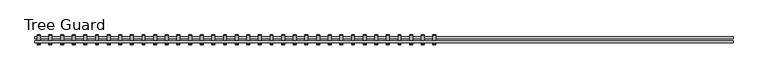
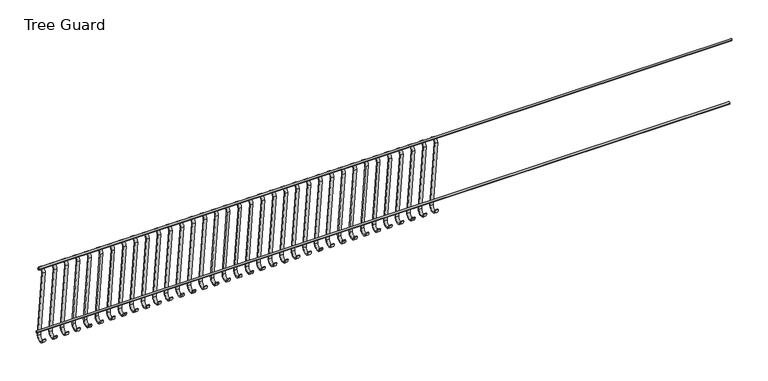
"""IFC4 building model written with IfcOpenShell, lengths in millimetres: railing geometry, Tree Guard."""

import ifcopenshell
import ifcopenshell.guid

model = None  # the IFC model being written
_history = None  # IfcOwnerHistory: only IFC2X3 demands one
_inside = {}  # id of a spatial element -> (the spatial element, [elements in it])
_under = {}  # id of a project, library or spatial element -> (it, [spatial elements below it])
_declared = {}  # id of a project -> (the project, [libraries it declares])
_typed = {}  # id of a type object -> (the type object, [elements of that type])
_made_of = {}  # id of a material, layer set ... -> (it, [elements and type objects made of it])


def new_model(schema):
    """Start an empty IFC model of exactly this schema.

    Asked for "IFC4X3", IfcOpenShell would pick the latest addendum, in which some entities
    have other attributes; the version numbers below select the first issue.
    IFC2X3 requires an IfcOwnerHistory on every rooted entity: one is made here for all.
    """
    global model, _history
    if schema == "IFC4X3":
        model = ifcopenshell.file(schema_version=(4, 3, 0, 0))
    else:
        model = ifcopenshell.file(schema=schema)
    _inside.clear()
    _under.clear()
    _declared.clear()
    _typed.clear()
    _made_of.clear()
    _history = None
    if model.schema == "IFC2X3":
        org = make("IfcOrganization", Name="unknown")
        user = make(
            "IfcPersonAndOrganization",
            ThePerson=make("IfcPerson", FamilyName="unknown"),
            TheOrganization=org,
        )
        app = make(
            "IfcApplication",
            ApplicationDeveloper=org,
            Version="unknown",
            ApplicationFullName="unknown",
            ApplicationIdentifier="unknown",
        )
        _history = make(
            "IfcOwnerHistory",
            OwningUser=user,
            OwningApplication=app,
            ChangeAction="ADDED",
            CreationDate=0,
        )
    return model


def make(cls, **values):
    """One entity of the class cls with the attributes given. An attribute that is None is left unset."""
    return model.create_entity(
        cls, **{name: value for name, value in values.items() if value is not None}
    )


def rooted(cls, **values):
    """An entity with a GlobalId (a new one), such as an element, a storey or a relation."""
    return make(cls, GlobalId=ifcopenshell.guid.new(), OwnerHistory=_history, **values)


def si_unit(unit_type, name, prefix=None):
    """IfcSIUnit, for example si_unit("LENGTHUNIT", "METRE", prefix="MILLI")."""
    return make("IfcSIUnit", UnitType=unit_type, Prefix=prefix, Name=name)


def assignment(units):
    """IfcUnitAssignment: the units of a project."""
    return None if units is None else make("IfcUnitAssignment", Units=units)


def point(xyz):
    """IfcCartesianPoint."""
    return None if xyz is None else make("IfcCartesianPoint", Coordinates=xyz)


def direction(xyz):
    """IfcDirection."""
    return None if xyz is None else make("IfcDirection", DirectionRatios=xyz)


def frame(location, z_axis=None, x_axis=None):
    """IfcAxis2Placement3D, a coordinate frame: its origin and axes. An axis left out is left unset."""
    return make(
        "IfcAxis2Placement3D",
        Location=point(location),
        Axis=direction(z_axis),
        RefDirection=direction(x_axis),
    )


def frame_2d(location, x_axis=None):
    """IfcAxis2Placement2D, a coordinate frame in the plane: its origin and x axis."""
    return make(
        "IfcAxis2Placement2D", Location=point(location), RefDirection=direction(x_axis)
    )


def origin():
    """The frame at (0, 0, 0) with its axes left unset."""
    return frame((0.0, 0.0, 0.0))


def place(relative_to, where):
    """IfcLocalPlacement: puts the frame where relative to a parent placement (None: the world)."""
    return make(
        "IfcLocalPlacement", PlacementRelTo=relative_to, RelativePlacement=where
    )


def context(
    kind, dimensions, precision=None, world=None, true_north=None, identifier=None
):
    """IfcGeometricRepresentationContext, for example the 3D "Model" context."""
    return make(
        "IfcGeometricRepresentationContext",
        ContextIdentifier=identifier,
        ContextType=kind,
        CoordinateSpaceDimension=dimensions,
        Precision=precision,
        WorldCoordinateSystem=world,
        TrueNorth=true_north,
    )


def project(units=None, contexts=None):
    """IfcProject with its units and contexts."""
    return rooted(
        "IfcProject",
        Name="project",
        RepresentationContexts=contexts,
        UnitsInContext=assignment(units),
    )


def spatial(cls, under=None, at=None, **own):
    """A site, building, storey or space (cls), placed at a placement, below another one or the project."""
    s = rooted(cls, ObjectPlacement=at, **own)
    if under is not None:
        _under.setdefault(under.id(), (under, []))[1].append(s)
    return s


def polyline(points):
    """IfcPolyline through the points."""
    return make("IfcPolyline", Points=[point(p) for p in points])


def circle_curve(where, radius):
    """IfcCircle in the frame where."""
    return make("IfcCircle", Position=where, Radius=radius)


def trimmed(basis, trim1, trim2, sense, master):
    """IfcTrimmedCurve: the piece of a basis curve between two trims."""
    return make(
        "IfcTrimmedCurve",
        BasisCurve=basis,
        Trim1=trim1,
        Trim2=trim2,
        SenseAgreement=sense,
        MasterRepresentation=master,
    )


def segment(curve, same_sense, transition):
    """IfcCompositeCurveSegment."""
    return make(
        "IfcCompositeCurveSegment",
        Transition=transition,
        SameSense=same_sense,
        ParentCurve=curve,
    )


def composite_curve(segments, self_intersect=None):
    """IfcCompositeCurve: segments joined end to end."""
    return make("IfcCompositeCurve", Segments=segments, SelfIntersect=self_intersect)


def outline(outer, holes=None, kind="AREA"):
    """IfcArbitraryClosedProfileDef: a profile drawn as a closed curve; with holes, ...WithVoids."""
    if holes is None:
        return make("IfcArbitraryClosedProfileDef", ProfileType=kind, OuterCurve=outer)
    return make(
        "IfcArbitraryProfileDefWithVoids",
        ProfileType=kind,
        OuterCurve=outer,
        InnerCurves=holes,
    )


def extrude(swept, where, along, depth):
    """IfcExtrudedAreaSolid: the profile swept, set in the frame where, extruded along a direction by depth."""
    return make(
        "IfcExtrudedAreaSolid",
        SweptArea=swept,
        Position=where,
        ExtrudedDirection=direction(along),
        Depth=depth,
    )


def shape(context_of_items, identifier, shape_type, items):
    """IfcShapeRepresentation: the items that make up one representation, for example the "Body"."""
    return make(
        "IfcShapeRepresentation",
        ContextOfItems=context_of_items,
        RepresentationIdentifier=identifier,
        RepresentationType=shape_type,
        Items=items,
    )


def source(mapping_origin, context_of_items, identifier, shape_type, items):
    """IfcRepresentationMap: a shape defined once, which mapped items show again and again."""
    return make(
        "IfcRepresentationMap",
        MappingOrigin=mapping_origin,
        MappedRepresentation=shape(context_of_items, identifier, shape_type, items),
    )


def transform(
    local_origin,
    x_axis=None,
    y_axis=None,
    z_axis=None,
    scale=None,
    scale2=None,
    scale3=None,
    uniform=True,
):
    """IfcCartesianTransformationOperator3D, or its non-uniform kind. x_axis, y_axis, z_axis: its Axis1, 2, 3."""
    if uniform:
        return make(
            "IfcCartesianTransformationOperator3D",
            Axis1=direction(x_axis),
            Axis2=direction(y_axis),
            LocalOrigin=point(local_origin),
            Scale=scale,
            Axis3=direction(z_axis),
        )
    return make(
        "IfcCartesianTransformationOperator3DnonUniform",
        Axis1=direction(x_axis),
        Axis2=direction(y_axis),
        LocalOrigin=point(local_origin),
        Scale=scale,
        Axis3=direction(z_axis),
        Scale2=scale2,
        Scale3=scale3,
    )


def mapped(mapping_source, mapping_target):
    """IfcMappedItem: shows the shape of a source again, moved by a transform."""
    return make(
        "IfcMappedItem", MappingSource=mapping_source, MappingTarget=mapping_target
    )


def made_of(thing, what):
    """Note that an element or type object is made of a material, layer set ...; save() writes the relation."""
    if what is not None:
        _made_of.setdefault(what.id(), (what, []))[1].append(thing)
    return thing


def element(
    cls,
    number,
    at=None,
    inside=None,
    cuts=None,
    type_object=None,
    material=None,
    context=None,
    identifier="Body",
    shape_type=None,
    held_by="IfcProductDefinitionShape",
    body=None,
    shapes=None,
    **own,
):
    """One element of the class cls, such as IfcWall. Its Tag is "e" and its number.

    at: its placement. inside: the storey or other place that contains it. cuts: it is an
    opening in that element (IfcRelVoidsElement). A single representation is given by context,
    identifier, shape_type and body (its items); several are given by shapes. held_by: the class
    of the entity that holds the representations. save() writes the other relations.
    """
    e = rooted(cls, Tag="e%d" % number, ObjectPlacement=at, **own)
    if body is not None:
        shapes = [shape(context, identifier, shape_type, body)]
    if shapes is not None:
        e.Representation = make(held_by, Representations=shapes)
    if inside is not None:
        _inside.setdefault(inside.id(), (inside, []))[1].append(e)
    if cuts is not None:
        rooted(
            "IfcRelVoidsElement", RelatingBuildingElement=cuts, RelatedOpeningElement=e
        )
    if type_object is not None:
        _typed.setdefault(type_object.id(), (type_object, []))[1].append(e)
    return made_of(e, material)


def aggregate(whole, parts):
    """IfcRelAggregates: a whole, such as a stair, and the parts it consists of."""
    return rooted("IfcRelAggregates", RelatingObject=whole, RelatedObjects=parts)


def save(model, path):
    """Write the relations noted so far, then the file.

    IfcRelAggregates (storeys below a building ...), IfcRelContainedInSpatialStructure (elements
    in a storey), IfcRelDefinesByType, IfcRelAssociatesMaterial and IfcRelDeclares: one each for
    every whole, place, type object, material and project.
    """
    for whole, parts in _under.values():
        aggregate(whole, parts)
    for where, things in _inside.values():
        rooted(
            "IfcRelContainedInSpatialStructure",
            RelatedElements=things,
            RelatingStructure=where,
        )
    for kind, things in _typed.values():
        rooted("IfcRelDefinesByType", RelatedObjects=things, RelatingType=kind)
    for what, things in _made_of.values():
        rooted("IfcRelAssociatesMaterial", RelatedObjects=things, RelatingMaterial=what)
    for by, libraries in _declared.values():
        rooted("IfcRelDeclares", RelatingContext=by, RelatedDefinitions=libraries)
    model.write(path)


def tree_guard_2ac65b3d(model_context):
    return source(origin(), model_context, "Body", "SweptSolid", [
        extrude(outline(composite_curve([segment(trimmed(circle_curve(frame_2d((-6583.9869829, 1054.1)), 12.7), [point((-6596.6869829, 1054.1))], [point((-6571.2869829, 1054.1))], False, "CARTESIAN"), True, "CONTINUOUS"), segment(trimmed(circle_curve(frame_2d((-6583.9869829, 1054.1)), 12.7), [point((-6571.2869829, 1054.1))], [point((-6596.6869829, 1054.1))], False, "CARTESIAN"), True, "CONTINUOUS")], self_intersect=False)), frame((-2784.641568, 0.0, 0.0), z_axis=(1.0, 0.0, 0.0), x_axis=(0.0, 1.0, 0.0)), (0.0, 0.0, 1.0), 9144.0),
        extrude(outline(composite_curve([segment(trimmed(circle_curve(frame_2d((-6533.1869829, 139.7)), 12.7), [point((-6545.8869829, 139.7))], [point((-6520.4869829, 139.7))], False, "CARTESIAN"), True, "CONTINUOUS"), segment(trimmed(circle_curve(frame_2d((-6533.1869829, 139.7)), 12.7), [point((-6520.4869829, 139.7))], [point((-6545.8869829, 139.7))], False, "CARTESIAN"), True, "CONTINUOUS")], self_intersect=False)), frame((-2784.641568, 0.0, 0.0), z_axis=(1.0, 0.0, 0.0), x_axis=(0.0, 1.0, 0.0)), (0.0, 0.0, 1.0), 9144.0),
        extrude(outline(composite_curve([segment(trimmed(circle_curve(frame_2d((-6558.5869829, 990.6)), 38.1), [point((-6520.4869829, 990.6))], [point((-6596.6815376, 991.2441257))], True, "CARTESIAN"), True, "CONTINUOUS"), segment(polyline([(-6596.6815376, 991.2441257), (-6495.0912061, 64.2323509)]), True, "CONTINUOUS"), segment(trimmed(circle_curve(frame_2d((-6558.5869829, 63.5)), 63.5), [point((-6495.0912061, 64.2323509))], [point((-6622.0869829, 63.5))], False, "CARTESIAN"), True, "CONTINUOUS"), segment(polyline([(-6622.0869829, 63.5), (-6609.3869829, 63.5)]), True, "CONTINUOUS"), segment(trimmed(circle_curve(frame_2d((-6558.5869829, 63.5)), 50.8), [point((-6609.3869829, 63.5))], [point((-6507.7869829, 63.5))], True, "CARTESIAN"), True, "CONTINUOUS"), segment(polyline([(-6507.7869829, 63.5), (-6609.3869829, 990.6)]), True, "CONTINUOUS"), segment(trimmed(circle_curve(frame_2d((-6558.5869829, 990.6)), 50.8), [point((-6609.3869829, 990.6))], [point((-6507.7869829, 990.6))], False, "CARTESIAN"), True, "CONTINUOUS"), segment(polyline([(-6507.7869829, 990.6), (-6520.4869829, 990.6)]), True, "CONTINUOUS")], self_intersect=False)), frame((-2752.891568, 0.0, 0.0), z_axis=(1.0, 0.0, 0.0), x_axis=(0.0, 1.0, 0.0)), (0.0, 0.0, 1.0), 38.1),
        extrude(outline(composite_curve([segment(trimmed(circle_curve(frame_2d((-6558.5869829, 990.6)), 38.1), [point((-6520.4869829, 990.6))], [point((-6596.6815376, 991.2441257))], True, "CARTESIAN"), True, "CONTINUOUS"), segment(polyline([(-6596.6815376, 991.2441257), (-6495.0912061, 64.2323509)]), True, "CONTINUOUS"), segment(trimmed(circle_curve(frame_2d((-6558.5869829, 63.5)), 63.5), [point((-6495.0912061, 64.2323509))], [point((-6622.0869829, 63.5))], False, "CARTESIAN"), True, "CONTINUOUS"), segment(polyline([(-6622.0869829, 63.5), (-6609.3869829, 63.5)]), True, "CONTINUOUS"), segment(trimmed(circle_curve(frame_2d((-6558.5869829, 63.5)), 50.8), [point((-6609.3869829, 63.5))], [point((-6507.7869829, 63.5))], True, "CARTESIAN"), True, "CONTINUOUS"), segment(polyline([(-6507.7869829, 63.5), (-6609.3869829, 990.6)]), True, "CONTINUOUS"), segment(trimmed(circle_curve(frame_2d((-6558.5869829, 990.6)), 50.8), [point((-6609.3869829, 990.6))], [point((-6507.7869829, 990.6))], False, "CARTESIAN"), True, "CONTINUOUS"), segment(polyline([(-6507.7869829, 990.6), (-6520.4869829, 990.6)]), True, "CONTINUOUS")], self_intersect=False)), frame((-2600.491568, 0.0, 0.0), z_axis=(1.0, 0.0, 0.0), x_axis=(0.0, 1.0, 0.0)), (0.0, 0.0, 1.0), 38.1),
        extrude(outline(composite_curve([segment(trimmed(circle_curve(frame_2d((-6558.5869829, 990.6)), 38.1), [point((-6520.4869829, 990.6))], [point((-6596.6815376, 991.2441257))], True, "CARTESIAN"), True, "CONTINUOUS"), segment(polyline([(-6596.6815376, 991.2441257), (-6495.0912061, 64.2323509)]), True, "CONTINUOUS"), segment(trimmed(circle_curve(frame_2d((-6558.5869829, 63.5)), 63.5), [point((-6495.0912061, 64.2323509))], [point((-6622.0869829, 63.5))], False, "CARTESIAN"), True, "CONTINUOUS"), segment(polyline([(-6622.0869829, 63.5), (-6609.3869829, 63.5)]), True, "CONTINUOUS"), segment(trimmed(circle_curve(frame_2d((-6558.5869829, 63.5)), 50.8), [point((-6609.3869829, 63.5))], [point((-6507.7869829, 63.5))], True, "CARTESIAN"), True, "CONTINUOUS"), segment(polyline([(-6507.7869829, 63.5), (-6609.3869829, 990.6)]), True, "CONTINUOUS"), segment(trimmed(circle_curve(frame_2d((-6558.5869829, 990.6)), 50.8), [point((-6609.3869829, 990.6))], [point((-6507.7869829, 990.6))], False, "CARTESIAN"), True, "CONTINUOUS"), segment(polyline([(-6507.7869829, 990.6), (-6520.4869829, 990.6)]), True, "CONTINUOUS")], self_intersect=False)), frame((-2448.091568, 0.0, 0.0), z_axis=(1.0, 0.0, 0.0), x_axis=(0.0, 1.0, 0.0)), (0.0, 0.0, 1.0), 38.1),
        extrude(outline(composite_curve([segment(trimmed(circle_curve(frame_2d((-6558.5869829, 990.6)), 38.1), [point((-6520.4869829, 990.6))], [point((-6596.6815376, 991.2441257))], True, "CARTESIAN"), True, "CONTINUOUS"), segment(polyline([(-6596.6815376, 991.2441257), (-6495.0912061, 64.2323509)]), True, "CONTINUOUS"), segment(trimmed(circle_curve(frame_2d((-6558.5869829, 63.5)), 63.5), [point((-6495.0912061, 64.2323509))], [point((-6622.0869829, 63.5))], False, "CARTESIAN"), True, "CONTINUOUS"), segment(polyline([(-6622.0869829, 63.5), (-6609.3869829, 63.5)]), True, "CONTINUOUS"), segment(trimmed(circle_curve(frame_2d((-6558.5869829, 63.5)), 50.8), [point((-6609.3869829, 63.5))], [point((-6507.7869829, 63.5))], True, "CARTESIAN"), True, "CONTINUOUS"), segment(polyline([(-6507.7869829, 63.5), (-6609.3869829, 990.6)]), True, "CONTINUOUS"), segment(trimmed(circle_curve(frame_2d((-6558.5869829, 990.6)), 50.8), [point((-6609.3869829, 990.6))], [point((-6507.7869829, 990.6))], False, "CARTESIAN"), True, "CONTINUOUS"), segment(polyline([(-6507.7869829, 990.6), (-6520.4869829, 990.6)]), True, "CONTINUOUS")], self_intersect=False)), frame((-2295.691568, 0.0, 0.0), z_axis=(1.0, 0.0, 0.0), x_axis=(0.0, 1.0, 0.0)), (0.0, 0.0, 1.0), 38.1),
        extrude(outline(composite_curve([segment(trimmed(circle_curve(frame_2d((-6558.5869829, 990.6)), 38.1), [point((-6520.4869829, 990.6))], [point((-6596.6815376, 991.2441257))], True, "CARTESIAN"), True, "CONTINUOUS"), segment(polyline([(-6596.6815376, 991.2441257), (-6495.0912061, 64.2323509)]), True, "CONTINUOUS"), segment(trimmed(circle_curve(frame_2d((-6558.5869829, 63.5)), 63.5), [point((-6495.0912061, 64.2323509))], [point((-6622.0869829, 63.5))], False, "CARTESIAN"), True, "CONTINUOUS"), segment(polyline([(-6622.0869829, 63.5), (-6609.3869829, 63.5)]), True, "CONTINUOUS"), segment(trimmed(circle_curve(frame_2d((-6558.5869829, 63.5)), 50.8), [point((-6609.3869829, 63.5))], [point((-6507.7869829, 63.5))], True, "CARTESIAN"), True, "CONTINUOUS"), segment(polyline([(-6507.7869829, 63.5), (-6609.3869829, 990.6)]), True, "CONTINUOUS"), segment(trimmed(circle_curve(frame_2d((-6558.5869829, 990.6)), 50.8), [point((-6609.3869829, 990.6))], [point((-6507.7869829, 990.6))], False, "CARTESIAN"), True, "CONTINUOUS"), segment(polyline([(-6507.7869829, 990.6), (-6520.4869829, 990.6)]), True, "CONTINUOUS")], self_intersect=False)), frame((-2143.291568, 0.0, 0.0), z_axis=(1.0, 0.0, 0.0), x_axis=(0.0, 1.0, 0.0)), (0.0, 0.0, 1.0), 38.1),
        extrude(outline(composite_curve([segment(trimmed(circle_curve(frame_2d((-6558.5869829, 990.6)), 38.1), [point((-6520.4869829, 990.6))], [point((-6596.6815376, 991.2441257))], True, "CARTESIAN"), True, "CONTINUOUS"), segment(polyline([(-6596.6815376, 991.2441257), (-6495.0912061, 64.2323509)]), True, "CONTINUOUS"), segment(trimmed(circle_curve(frame_2d((-6558.5869829, 63.5)), 63.5), [point((-6495.0912061, 64.2323509))], [point((-6622.0869829, 63.5))], False, "CARTESIAN"), True, "CONTINUOUS"), segment(polyline([(-6622.0869829, 63.5), (-6609.3869829, 63.5)]), True, "CONTINUOUS"), segment(trimmed(circle_curve(frame_2d((-6558.5869829, 63.5)), 50.8), [point((-6609.3869829, 63.5))], [point((-6507.7869829, 63.5))], True, "CARTESIAN"), True, "CONTINUOUS"), segment(polyline([(-6507.7869829, 63.5), (-6609.3869829, 990.6)]), True, "CONTINUOUS"), segment(trimmed(circle_curve(frame_2d((-6558.5869829, 990.6)), 50.8), [point((-6609.3869829, 990.6))], [point((-6507.7869829, 990.6))], False, "CARTESIAN"), True, "CONTINUOUS"), segment(polyline([(-6507.7869829, 990.6), (-6520.4869829, 990.6)]), True, "CONTINUOUS")], self_intersect=False)), frame((-1990.891568, 0.0, 0.0), z_axis=(1.0, 0.0, 0.0), x_axis=(0.0, 1.0, 0.0)), (0.0, 0.0, 1.0), 38.1),
        extrude(outline(composite_curve([segment(trimmed(circle_curve(frame_2d((-6558.5869829, 990.6)), 38.1), [point((-6520.4869829, 990.6))], [point((-6596.6815376, 991.2441257))], True, "CARTESIAN"), True, "CONTINUOUS"), segment(polyline([(-6596.6815376, 991.2441257), (-6495.0912061, 64.2323509)]), True, "CONTINUOUS"), segment(trimmed(circle_curve(frame_2d((-6558.5869829, 63.5)), 63.5), [point((-6495.0912061, 64.2323509))], [point((-6622.0869829, 63.5))], False, "CARTESIAN"), True, "CONTINUOUS"), segment(polyline([(-6622.0869829, 63.5), (-6609.3869829, 63.5)]), True, "CONTINUOUS"), segment(trimmed(circle_curve(frame_2d((-6558.5869829, 63.5)), 50.8), [point((-6609.3869829, 63.5))], [point((-6507.7869829, 63.5))], True, "CARTESIAN"), True, "CONTINUOUS"), segment(polyline([(-6507.7869829, 63.5), (-6609.3869829, 990.6)]), True, "CONTINUOUS"), segment(trimmed(circle_curve(frame_2d((-6558.5869829, 990.6)), 50.8), [point((-6609.3869829, 990.6))], [point((-6507.7869829, 990.6))], False, "CARTESIAN"), True, "CONTINUOUS"), segment(polyline([(-6507.7869829, 990.6), (-6520.4869829, 990.6)]), True, "CONTINUOUS")], self_intersect=False)), frame((-1838.491568, 0.0, 0.0), z_axis=(1.0, 0.0, 0.0), x_axis=(0.0, 1.0, 0.0)), (0.0, 0.0, 1.0), 38.1),
        extrude(outline(composite_curve([segment(trimmed(circle_curve(frame_2d((-6558.5869829, 990.6)), 38.1), [point((-6520.4869829, 990.6))], [point((-6596.6815376, 991.2441257))], True, "CARTESIAN"), True, "CONTINUOUS"), segment(polyline([(-6596.6815376, 991.2441257), (-6495.0912061, 64.2323509)]), True, "CONTINUOUS"), segment(trimmed(circle_curve(frame_2d((-6558.5869829, 63.5)), 63.5), [point((-6495.0912061, 64.2323509))], [point((-6622.0869829, 63.5))], False, "CARTESIAN"), True, "CONTINUOUS"), segment(polyline([(-6622.0869829, 63.5), (-6609.3869829, 63.5)]), True, "CONTINUOUS"), segment(trimmed(circle_curve(frame_2d((-6558.5869829, 63.5)), 50.8), [point((-6609.3869829, 63.5))], [point((-6507.7869829, 63.5))], True, "CARTESIAN"), True, "CONTINUOUS"), segment(polyline([(-6507.7869829, 63.5), (-6609.3869829, 990.6)]), True, "CONTINUOUS"), segment(trimmed(circle_curve(frame_2d((-6558.5869829, 990.6)), 50.8), [point((-6609.3869829, 990.6))], [point((-6507.7869829, 990.6))], False, "CARTESIAN"), True, "CONTINUOUS"), segment(polyline([(-6507.7869829, 990.6), (-6520.4869829, 990.6)]), True, "CONTINUOUS")], self_intersect=False)), frame((-1686.091568, 0.0, 0.0), z_axis=(1.0, 0.0, 0.0), x_axis=(0.0, 1.0, 0.0)), (0.0, 0.0, 1.0), 38.1),
        extrude(outline(composite_curve([segment(trimmed(circle_curve(frame_2d((-6558.5869829, 990.6)), 38.1), [point((-6520.4869829, 990.6))], [point((-6596.6815376, 991.2441257))], True, "CARTESIAN"), True, "CONTINUOUS"), segment(polyline([(-6596.6815376, 991.2441257), (-6495.0912061, 64.2323509)]), True, "CONTINUOUS"), segment(trimmed(circle_curve(frame_2d((-6558.5869829, 63.5)), 63.5), [point((-6495.0912061, 64.2323509))], [point((-6622.0869829, 63.5))], False, "CARTESIAN"), True, "CONTINUOUS"), segment(polyline([(-6622.0869829, 63.5), (-6609.3869829, 63.5)]), True, "CONTINUOUS"), segment(trimmed(circle_curve(frame_2d((-6558.5869829, 63.5)), 50.8), [point((-6609.3869829, 63.5))], [point((-6507.7869829, 63.5))], True, "CARTESIAN"), True, "CONTINUOUS"), segment(polyline([(-6507.7869829, 63.5), (-6609.3869829, 990.6)]), True, "CONTINUOUS"), segment(trimmed(circle_curve(frame_2d((-6558.5869829, 990.6)), 50.8), [point((-6609.3869829, 990.6))], [point((-6507.7869829, 990.6))], False, "CARTESIAN"), True, "CONTINUOUS"), segment(polyline([(-6507.7869829, 990.6), (-6520.4869829, 990.6)]), True, "CONTINUOUS")], self_intersect=False)), frame((-1533.691568, 0.0, 0.0), z_axis=(1.0, 0.0, 0.0), x_axis=(0.0, 1.0, 0.0)), (0.0, 0.0, 1.0), 38.1),
        extrude(outline(composite_curve([segment(trimmed(circle_curve(frame_2d((-6558.5869829, 990.6)), 38.1), [point((-6520.4869829, 990.6))], [point((-6596.6815376, 991.2441257))], True, "CARTESIAN"), True, "CONTINUOUS"), segment(polyline([(-6596.6815376, 991.2441257), (-6495.0912061, 64.2323509)]), True, "CONTINUOUS"), segment(trimmed(circle_curve(frame_2d((-6558.5869829, 63.5)), 63.5), [point((-6495.0912061, 64.2323509))], [point((-6622.0869829, 63.5))], False, "CARTESIAN"), True, "CONTINUOUS"), segment(polyline([(-6622.0869829, 63.5), (-6609.3869829, 63.5)]), True, "CONTINUOUS"), segment(trimmed(circle_curve(frame_2d((-6558.5869829, 63.5)), 50.8), [point((-6609.3869829, 63.5))], [point((-6507.7869829, 63.5))], True, "CARTESIAN"), True, "CONTINUOUS"), segment(polyline([(-6507.7869829, 63.5), (-6609.3869829, 990.6)]), True, "CONTINUOUS"), segment(trimmed(circle_curve(frame_2d((-6558.5869829, 990.6)), 50.8), [point((-6609.3869829, 990.6))], [point((-6507.7869829, 990.6))], False, "CARTESIAN"), True, "CONTINUOUS"), segment(polyline([(-6507.7869829, 990.6), (-6520.4869829, 990.6)]), True, "CONTINUOUS")], self_intersect=False)), frame((-1381.291568, 0.0, 0.0), z_axis=(1.0, 0.0, 0.0), x_axis=(0.0, 1.0, 0.0)), (0.0, 0.0, 1.0), 38.1),
        extrude(outline(composite_curve([segment(trimmed(circle_curve(frame_2d((-6558.5869829, 990.6)), 38.1), [point((-6520.4869829, 990.6))], [point((-6596.6815376, 991.2441257))], True, "CARTESIAN"), True, "CONTINUOUS"), segment(polyline([(-6596.6815376, 991.2441257), (-6495.0912061, 64.2323509)]), True, "CONTINUOUS"), segment(trimmed(circle_curve(frame_2d((-6558.5869829, 63.5)), 63.5), [point((-6495.0912061, 64.2323509))], [point((-6622.0869829, 63.5))], False, "CARTESIAN"), True, "CONTINUOUS"), segment(polyline([(-6622.0869829, 63.5), (-6609.3869829, 63.5)]), True, "CONTINUOUS"), segment(trimmed(circle_curve(frame_2d((-6558.5869829, 63.5)), 50.8), [point((-6609.3869829, 63.5))], [point((-6507.7869829, 63.5))], True, "CARTESIAN"), True, "CONTINUOUS"), segment(polyline([(-6507.7869829, 63.5), (-6609.3869829, 990.6)]), True, "CONTINUOUS"), segment(trimmed(circle_curve(frame_2d((-6558.5869829, 990.6)), 50.8), [point((-6609.3869829, 990.6))], [point((-6507.7869829, 990.6))], False, "CARTESIAN"), True, "CONTINUOUS"), segment(polyline([(-6507.7869829, 990.6), (-6520.4869829, 990.6)]), True, "CONTINUOUS")], self_intersect=False)), frame((-1228.891568, 0.0, 0.0), z_axis=(1.0, 0.0, 0.0), x_axis=(0.0, 1.0, 0.0)), (0.0, 0.0, 1.0), 38.1),
        extrude(outline(composite_curve([segment(trimmed(circle_curve(frame_2d((-6558.5869829, 990.6)), 38.1), [point((-6520.4869829, 990.6))], [point((-6596.6815376, 991.2441257))], True, "CARTESIAN"), True, "CONTINUOUS"), segment(polyline([(-6596.6815376, 991.2441257), (-6495.0912061, 64.2323509)]), True, "CONTINUOUS"), segment(trimmed(circle_curve(frame_2d((-6558.5869829, 63.5)), 63.5), [point((-6495.0912061, 64.2323509))], [point((-6622.0869829, 63.5))], False, "CARTESIAN"), True, "CONTINUOUS"), segment(polyline([(-6622.0869829, 63.5), (-6609.3869829, 63.5)]), True, "CONTINUOUS"), segment(trimmed(circle_curve(frame_2d((-6558.5869829, 63.5)), 50.8), [point((-6609.3869829, 63.5))], [point((-6507.7869829, 63.5))], True, "CARTESIAN"), True, "CONTINUOUS"), segment(polyline([(-6507.7869829, 63.5), (-6609.3869829, 990.6)]), True, "CONTINUOUS"), segment(trimmed(circle_curve(frame_2d((-6558.5869829, 990.6)), 50.8), [point((-6609.3869829, 990.6))], [point((-6507.7869829, 990.6))], False, "CARTESIAN"), True, "CONTINUOUS"), segment(polyline([(-6507.7869829, 990.6), (-6520.4869829, 990.6)]), True, "CONTINUOUS")], self_intersect=False)), frame((-1076.491568, 0.0, 0.0), z_axis=(1.0, 0.0, 0.0), x_axis=(0.0, 1.0, 0.0)), (0.0, 0.0, 1.0), 38.1),
        extrude(outline(composite_curve([segment(trimmed(circle_curve(frame_2d((-6558.5869829, 990.6)), 38.1), [point((-6520.4869829, 990.6))], [point((-6596.6815376, 991.2441257))], True, "CARTESIAN"), True, "CONTINUOUS"), segment(polyline([(-6596.6815376, 991.2441257), (-6495.0912061, 64.2323509)]), True, "CONTINUOUS"), segment(trimmed(circle_curve(frame_2d((-6558.5869829, 63.5)), 63.5), [point((-6495.0912061, 64.2323509))], [point((-6622.0869829, 63.5))], False, "CARTESIAN"), True, "CONTINUOUS"), segment(polyline([(-6622.0869829, 63.5), (-6609.3869829, 63.5)]), True, "CONTINUOUS"), segment(trimmed(circle_curve(frame_2d((-6558.5869829, 63.5)), 50.8), [point((-6609.3869829, 63.5))], [point((-6507.7869829, 63.5))], True, "CARTESIAN"), True, "CONTINUOUS"), segment(polyline([(-6507.7869829, 63.5), (-6609.3869829, 990.6)]), True, "CONTINUOUS"), segment(trimmed(circle_curve(frame_2d((-6558.5869829, 990.6)), 50.8), [point((-6609.3869829, 990.6))], [point((-6507.7869829, 990.6))], False, "CARTESIAN"), True, "CONTINUOUS"), segment(polyline([(-6507.7869829, 990.6), (-6520.4869829, 990.6)]), True, "CONTINUOUS")], self_intersect=False)), frame((-924.091568, 0.0, 0.0), z_axis=(1.0, 0.0, 0.0), x_axis=(0.0, 1.0, 0.0)), (0.0, 0.0, 1.0), 38.1),
        extrude(outline(composite_curve([segment(trimmed(circle_curve(frame_2d((-6558.5869829, 990.6)), 38.1), [point((-6520.4869829, 990.6))], [point((-6596.6815376, 991.2441257))], True, "CARTESIAN"), True, "CONTINUOUS"), segment(polyline([(-6596.6815376, 991.2441257), (-6495.0912061, 64.2323509)]), True, "CONTINUOUS"), segment(trimmed(circle_curve(frame_2d((-6558.5869829, 63.5)), 63.5), [point((-6495.0912061, 64.2323509))], [point((-6622.0869829, 63.5))], False, "CARTESIAN"), True, "CONTINUOUS"), segment(polyline([(-6622.0869829, 63.5), (-6609.3869829, 63.5)]), True, "CONTINUOUS"), segment(trimmed(circle_curve(frame_2d((-6558.5869829, 63.5)), 50.8), [point((-6609.3869829, 63.5))], [point((-6507.7869829, 63.5))], True, "CARTESIAN"), True, "CONTINUOUS"), segment(polyline([(-6507.7869829, 63.5), (-6609.3869829, 990.6)]), True, "CONTINUOUS"), segment(trimmed(circle_curve(frame_2d((-6558.5869829, 990.6)), 50.8), [point((-6609.3869829, 990.6))], [point((-6507.7869829, 990.6))], False, "CARTESIAN"), True, "CONTINUOUS"), segment(polyline([(-6507.7869829, 990.6), (-6520.4869829, 990.6)]), True, "CONTINUOUS")], self_intersect=False)), frame((-771.691568, 0.0, 0.0), z_axis=(1.0, 0.0, 0.0), x_axis=(0.0, 1.0, 0.0)), (0.0, 0.0, 1.0), 38.1),
        extrude(outline(composite_curve([segment(trimmed(circle_curve(frame_2d((-6558.5869829, 990.6)), 38.1), [point((-6520.4869829, 990.6))], [point((-6596.6815376, 991.2441257))], True, "CARTESIAN"), True, "CONTINUOUS"), segment(polyline([(-6596.6815376, 991.2441257), (-6495.0912061, 64.2323509)]), True, "CONTINUOUS"), segment(trimmed(circle_curve(frame_2d((-6558.5869829, 63.5)), 63.5), [point((-6495.0912061, 64.2323509))], [point((-6622.0869829, 63.5))], False, "CARTESIAN"), True, "CONTINUOUS"), segment(polyline([(-6622.0869829, 63.5), (-6609.3869829, 63.5)]), True, "CONTINUOUS"), segment(trimmed(circle_curve(frame_2d((-6558.5869829, 63.5)), 50.8), [point((-6609.3869829, 63.5))], [point((-6507.7869829, 63.5))], True, "CARTESIAN"), True, "CONTINUOUS"), segment(polyline([(-6507.7869829, 63.5), (-6609.3869829, 990.6)]), True, "CONTINUOUS"), segment(trimmed(circle_curve(frame_2d((-6558.5869829, 990.6)), 50.8), [point((-6609.3869829, 990.6))], [point((-6507.7869829, 990.6))], False, "CARTESIAN"), True, "CONTINUOUS"), segment(polyline([(-6507.7869829, 990.6), (-6520.4869829, 990.6)]), True, "CONTINUOUS")], self_intersect=False)), frame((-619.291568, 0.0, 0.0), z_axis=(1.0, 0.0, 0.0), x_axis=(0.0, 1.0, 0.0)), (0.0, 0.0, 1.0), 38.1),
        extrude(outline(composite_curve([segment(trimmed(circle_curve(frame_2d((-6558.5869829, 990.6)), 38.1), [point((-6520.4869829, 990.6))], [point((-6596.6815376, 991.2441257))], True, "CARTESIAN"), True, "CONTINUOUS"), segment(polyline([(-6596.6815376, 991.2441257), (-6495.0912061, 64.2323509)]), True, "CONTINUOUS"), segment(trimmed(circle_curve(frame_2d((-6558.5869829, 63.5)), 63.5), [point((-6495.0912061, 64.2323509))], [point((-6622.0869829, 63.5))], False, "CARTESIAN"), True, "CONTINUOUS"), segment(polyline([(-6622.0869829, 63.5), (-6609.3869829, 63.5)]), True, "CONTINUOUS"), segment(trimmed(circle_curve(frame_2d((-6558.5869829, 63.5)), 50.8), [point((-6609.3869829, 63.5))], [point((-6507.7869829, 63.5))], True, "CARTESIAN"), True, "CONTINUOUS"), segment(polyline([(-6507.7869829, 63.5), (-6609.3869829, 990.6)]), True, "CONTINUOUS"), segment(trimmed(circle_curve(frame_2d((-6558.5869829, 990.6)), 50.8), [point((-6609.3869829, 990.6))], [point((-6507.7869829, 990.6))], False, "CARTESIAN"), True, "CONTINUOUS"), segment(polyline([(-6507.7869829, 990.6), (-6520.4869829, 990.6)]), True, "CONTINUOUS")], self_intersect=False)), frame((-466.891568, 0.0, 0.0), z_axis=(1.0, 0.0, 0.0), x_axis=(0.0, 1.0, 0.0)), (0.0, 0.0, 1.0), 38.1),
        extrude(outline(composite_curve([segment(trimmed(circle_curve(frame_2d((-6558.5869829, 990.6)), 38.1), [point((-6520.4869829, 990.6))], [point((-6596.6815376, 991.2441257))], True, "CARTESIAN"), True, "CONTINUOUS"), segment(polyline([(-6596.6815376, 991.2441257), (-6495.0912061, 64.2323509)]), True, "CONTINUOUS"), segment(trimmed(circle_curve(frame_2d((-6558.5869829, 63.5)), 63.5), [point((-6495.0912061, 64.2323509))], [point((-6622.0869829, 63.5))], False, "CARTESIAN"), True, "CONTINUOUS"), segment(polyline([(-6622.0869829, 63.5), (-6609.3869829, 63.5)]), True, "CONTINUOUS"), segment(trimmed(circle_curve(frame_2d((-6558.5869829, 63.5)), 50.8), [point((-6609.3869829, 63.5))], [point((-6507.7869829, 63.5))], True, "CARTESIAN"), True, "CONTINUOUS"), segment(polyline([(-6507.7869829, 63.5), (-6609.3869829, 990.6)]), True, "CONTINUOUS"), segment(trimmed(circle_curve(frame_2d((-6558.5869829, 990.6)), 50.8), [point((-6609.3869829, 990.6))], [point((-6507.7869829, 990.6))], False, "CARTESIAN"), True, "CONTINUOUS"), segment(polyline([(-6507.7869829, 990.6), (-6520.4869829, 990.6)]), True, "CONTINUOUS")], self_intersect=False)), frame((-314.491568, 0.0, 0.0), z_axis=(1.0, 0.0, 0.0), x_axis=(0.0, 1.0, 0.0)), (0.0, 0.0, 1.0), 38.1),
        extrude(outline(composite_curve([segment(trimmed(circle_curve(frame_2d((-6558.5869829, 990.6)), 38.1), [point((-6520.4869829, 990.6))], [point((-6596.6815376, 991.2441257))], True, "CARTESIAN"), True, "CONTINUOUS"), segment(polyline([(-6596.6815376, 991.2441257), (-6495.0912061, 64.2323509)]), True, "CONTINUOUS"), segment(trimmed(circle_curve(frame_2d((-6558.5869829, 63.5)), 63.5), [point((-6495.0912061, 64.2323509))], [point((-6622.0869829, 63.5))], False, "CARTESIAN"), True, "CONTINUOUS"), segment(polyline([(-6622.0869829, 63.5), (-6609.3869829, 63.5)]), True, "CONTINUOUS"), segment(trimmed(circle_curve(frame_2d((-6558.5869829, 63.5)), 50.8), [point((-6609.3869829, 63.5))], [point((-6507.7869829, 63.5))], True, "CARTESIAN"), True, "CONTINUOUS"), segment(polyline([(-6507.7869829, 63.5), (-6609.3869829, 990.6)]), True, "CONTINUOUS"), segment(trimmed(circle_curve(frame_2d((-6558.5869829, 990.6)), 50.8), [point((-6609.3869829, 990.6))], [point((-6507.7869829, 990.6))], False, "CARTESIAN"), True, "CONTINUOUS"), segment(polyline([(-6507.7869829, 990.6), (-6520.4869829, 990.6)]), True, "CONTINUOUS")], self_intersect=False)), frame((-162.091568, 0.0, 0.0), z_axis=(1.0, 0.0, 0.0), x_axis=(0.0, 1.0, 0.0)), (0.0, 0.0, 1.0), 38.1),
        extrude(outline(composite_curve([segment(trimmed(circle_curve(frame_2d((-6558.5869829, 990.6)), 38.1), [point((-6520.4869829, 990.6))], [point((-6596.6815376, 991.2441257))], True, "CARTESIAN"), True, "CONTINUOUS"), segment(polyline([(-6596.6815376, 991.2441257), (-6495.0912061, 64.2323509)]), True, "CONTINUOUS"), segment(trimmed(circle_curve(frame_2d((-6558.5869829, 63.5)), 63.5), [point((-6495.0912061, 64.2323509))], [point((-6622.0869829, 63.5))], False, "CARTESIAN"), True, "CONTINUOUS"), segment(polyline([(-6622.0869829, 63.5), (-6609.3869829, 63.5)]), True, "CONTINUOUS"), segment(trimmed(circle_curve(frame_2d((-6558.5869829, 63.5)), 50.8), [point((-6609.3869829, 63.5))], [point((-6507.7869829, 63.5))], True, "CARTESIAN"), True, "CONTINUOUS"), segment(polyline([(-6507.7869829, 63.5), (-6609.3869829, 990.6)]), True, "CONTINUOUS"), segment(trimmed(circle_curve(frame_2d((-6558.5869829, 990.6)), 50.8), [point((-6609.3869829, 990.6))], [point((-6507.7869829, 990.6))], False, "CARTESIAN"), True, "CONTINUOUS"), segment(polyline([(-6507.7869829, 990.6), (-6520.4869829, 990.6)]), True, "CONTINUOUS")], self_intersect=False)), frame((-9.691568, 0.0, 0.0), z_axis=(1.0, 0.0, 0.0), x_axis=(0.0, 1.0, 0.0)), (0.0, 0.0, 1.0), 38.1),
        extrude(outline(composite_curve([segment(trimmed(circle_curve(frame_2d((-6558.5869829, 990.6)), 38.1), [point((-6520.4869829, 990.6))], [point((-6596.6815376, 991.2441257))], True, "CARTESIAN"), True, "CONTINUOUS"), segment(polyline([(-6596.6815376, 991.2441257), (-6495.0912061, 64.2323509)]), True, "CONTINUOUS"), segment(trimmed(circle_curve(frame_2d((-6558.5869829, 63.5)), 63.5), [point((-6495.0912061, 64.2323509))], [point((-6622.0869829, 63.5))], False, "CARTESIAN"), True, "CONTINUOUS"), segment(polyline([(-6622.0869829, 63.5), (-6609.3869829, 63.5)]), True, "CONTINUOUS"), segment(trimmed(circle_curve(frame_2d((-6558.5869829, 63.5)), 50.8), [point((-6609.3869829, 63.5))], [point((-6507.7869829, 63.5))], True, "CARTESIAN"), True, "CONTINUOUS"), segment(polyline([(-6507.7869829, 63.5), (-6609.3869829, 990.6)]), True, "CONTINUOUS"), segment(trimmed(circle_curve(frame_2d((-6558.5869829, 990.6)), 50.8), [point((-6609.3869829, 990.6))], [point((-6507.7869829, 990.6))], False, "CARTESIAN"), True, "CONTINUOUS"), segment(polyline([(-6507.7869829, 990.6), (-6520.4869829, 990.6)]), True, "CONTINUOUS")], self_intersect=False)), frame((142.708432, 0.0, 0.0), z_axis=(1.0, 0.0, 0.0), x_axis=(0.0, 1.0, 0.0)), (0.0, 0.0, 1.0), 38.1),
        extrude(outline(composite_curve([segment(trimmed(circle_curve(frame_2d((-6558.5869829, 990.6)), 38.1), [point((-6520.4869829, 990.6))], [point((-6596.6815376, 991.2441257))], True, "CARTESIAN"), True, "CONTINUOUS"), segment(polyline([(-6596.6815376, 991.2441257), (-6495.0912061, 64.2323509)]), True, "CONTINUOUS"), segment(trimmed(circle_curve(frame_2d((-6558.5869829, 63.5)), 63.5), [point((-6495.0912061, 64.2323509))], [point((-6622.0869829, 63.5))], False, "CARTESIAN"), True, "CONTINUOUS"), segment(polyline([(-6622.0869829, 63.5), (-6609.3869829, 63.5)]), True, "CONTINUOUS"), segment(trimmed(circle_curve(frame_2d((-6558.5869829, 63.5)), 50.8), [point((-6609.3869829, 63.5))], [point((-6507.7869829, 63.5))], True, "CARTESIAN"), True, "CONTINUOUS"), segment(polyline([(-6507.7869829, 63.5), (-6609.3869829, 990.6)]), True, "CONTINUOUS"), segment(trimmed(circle_curve(frame_2d((-6558.5869829, 990.6)), 50.8), [point((-6609.3869829, 990.6))], [point((-6507.7869829, 990.6))], False, "CARTESIAN"), True, "CONTINUOUS"), segment(polyline([(-6507.7869829, 990.6), (-6520.4869829, 990.6)]), True, "CONTINUOUS")], self_intersect=False)), frame((295.108432, 0.0, 0.0), z_axis=(1.0, 0.0, 0.0), x_axis=(0.0, 1.0, 0.0)), (0.0, 0.0, 1.0), 38.1),
        extrude(outline(composite_curve([segment(trimmed(circle_curve(frame_2d((-6558.5869829, 990.6)), 38.1), [point((-6520.4869829, 990.6))], [point((-6596.6815376, 991.2441257))], True, "CARTESIAN"), True, "CONTINUOUS"), segment(polyline([(-6596.6815376, 991.2441257), (-6495.0912061, 64.2323509)]), True, "CONTINUOUS"), segment(trimmed(circle_curve(frame_2d((-6558.5869829, 63.5)), 63.5), [point((-6495.0912061, 64.2323509))], [point((-6622.0869829, 63.5))], False, "CARTESIAN"), True, "CONTINUOUS"), segment(polyline([(-6622.0869829, 63.5), (-6609.3869829, 63.5)]), True, "CONTINUOUS"), segment(trimmed(circle_curve(frame_2d((-6558.5869829, 63.5)), 50.8), [point((-6609.3869829, 63.5))], [point((-6507.7869829, 63.5))], True, "CARTESIAN"), True, "CONTINUOUS"), segment(polyline([(-6507.7869829, 63.5), (-6609.3869829, 990.6)]), True, "CONTINUOUS"), segment(trimmed(circle_curve(frame_2d((-6558.5869829, 990.6)), 50.8), [point((-6609.3869829, 990.6))], [point((-6507.7869829, 990.6))], False, "CARTESIAN"), True, "CONTINUOUS"), segment(polyline([(-6507.7869829, 990.6), (-6520.4869829, 990.6)]), True, "CONTINUOUS")], self_intersect=False)), frame((447.508432, 0.0, 0.0), z_axis=(1.0, 0.0, 0.0), x_axis=(0.0, 1.0, 0.0)), (0.0, 0.0, 1.0), 38.1),
        extrude(outline(composite_curve([segment(trimmed(circle_curve(frame_2d((-6558.5869829, 990.6)), 38.1), [point((-6520.4869829, 990.6))], [point((-6596.6815376, 991.2441257))], True, "CARTESIAN"), True, "CONTINUOUS"), segment(polyline([(-6596.6815376, 991.2441257), (-6495.0912061, 64.2323509)]), True, "CONTINUOUS"), segment(trimmed(circle_curve(frame_2d((-6558.5869829, 63.5)), 63.5), [point((-6495.0912061, 64.2323509))], [point((-6622.0869829, 63.5))], False, "CARTESIAN"), True, "CONTINUOUS"), segment(polyline([(-6622.0869829, 63.5), (-6609.3869829, 63.5)]), True, "CONTINUOUS"), segment(trimmed(circle_curve(frame_2d((-6558.5869829, 63.5)), 50.8), [point((-6609.3869829, 63.5))], [point((-6507.7869829, 63.5))], True, "CARTESIAN"), True, "CONTINUOUS"), segment(polyline([(-6507.7869829, 63.5), (-6609.3869829, 990.6)]), True, "CONTINUOUS"), segment(trimmed(circle_curve(frame_2d((-6558.5869829, 990.6)), 50.8), [point((-6609.3869829, 990.6))], [point((-6507.7869829, 990.6))], False, "CARTESIAN"), True, "CONTINUOUS"), segment(polyline([(-6507.7869829, 990.6), (-6520.4869829, 990.6)]), True, "CONTINUOUS")], self_intersect=False)), frame((599.908432, 0.0, 0.0), z_axis=(1.0, 0.0, 0.0), x_axis=(0.0, 1.0, 0.0)), (0.0, 0.0, 1.0), 38.1),
        extrude(outline(composite_curve([segment(trimmed(circle_curve(frame_2d((-6558.5869829, 990.6)), 38.1), [point((-6520.4869829, 990.6))], [point((-6596.6815376, 991.2441257))], True, "CARTESIAN"), True, "CONTINUOUS"), segment(polyline([(-6596.6815376, 991.2441257), (-6495.0912061, 64.2323509)]), True, "CONTINUOUS"), segment(trimmed(circle_curve(frame_2d((-6558.5869829, 63.5)), 63.5), [point((-6495.0912061, 64.2323509))], [point((-6622.0869829, 63.5))], False, "CARTESIAN"), True, "CONTINUOUS"), segment(polyline([(-6622.0869829, 63.5), (-6609.3869829, 63.5)]), True, "CONTINUOUS"), segment(trimmed(circle_curve(frame_2d((-6558.5869829, 63.5)), 50.8), [point((-6609.3869829, 63.5))], [point((-6507.7869829, 63.5))], True, "CARTESIAN"), True, "CONTINUOUS"), segment(polyline([(-6507.7869829, 63.5), (-6609.3869829, 990.6)]), True, "CONTINUOUS"), segment(trimmed(circle_curve(frame_2d((-6558.5869829, 990.6)), 50.8), [point((-6609.3869829, 990.6))], [point((-6507.7869829, 990.6))], False, "CARTESIAN"), True, "CONTINUOUS"), segment(polyline([(-6507.7869829, 990.6), (-6520.4869829, 990.6)]), True, "CONTINUOUS")], self_intersect=False)), frame((752.308432, 0.0, 0.0), z_axis=(1.0, 0.0, 0.0), x_axis=(0.0, 1.0, 0.0)), (0.0, 0.0, 1.0), 38.1),
        extrude(outline(composite_curve([segment(trimmed(circle_curve(frame_2d((-6558.5869829, 990.6)), 38.1), [point((-6520.4869829, 990.6))], [point((-6596.6815376, 991.2441257))], True, "CARTESIAN"), True, "CONTINUOUS"), segment(polyline([(-6596.6815376, 991.2441257), (-6495.0912061, 64.2323509)]), True, "CONTINUOUS"), segment(trimmed(circle_curve(frame_2d((-6558.5869829, 63.5)), 63.5), [point((-6495.0912061, 64.2323509))], [point((-6622.0869829, 63.5))], False, "CARTESIAN"), True, "CONTINUOUS"), segment(polyline([(-6622.0869829, 63.5), (-6609.3869829, 63.5)]), True, "CONTINUOUS"), segment(trimmed(circle_curve(frame_2d((-6558.5869829, 63.5)), 50.8), [point((-6609.3869829, 63.5))], [point((-6507.7869829, 63.5))], True, "CARTESIAN"), True, "CONTINUOUS"), segment(polyline([(-6507.7869829, 63.5), (-6609.3869829, 990.6)]), True, "CONTINUOUS"), segment(trimmed(circle_curve(frame_2d((-6558.5869829, 990.6)), 50.8), [point((-6609.3869829, 990.6))], [point((-6507.7869829, 990.6))], False, "CARTESIAN"), True, "CONTINUOUS"), segment(polyline([(-6507.7869829, 990.6), (-6520.4869829, 990.6)]), True, "CONTINUOUS")], self_intersect=False)), frame((904.708432, 0.0, 0.0), z_axis=(1.0, 0.0, 0.0), x_axis=(0.0, 1.0, 0.0)), (0.0, 0.0, 1.0), 38.1),
        extrude(outline(composite_curve([segment(trimmed(circle_curve(frame_2d((-6558.5869829, 990.6)), 38.1), [point((-6520.4869829, 990.6))], [point((-6596.6815376, 991.2441257))], True, "CARTESIAN"), True, "CONTINUOUS"), segment(polyline([(-6596.6815376, 991.2441257), (-6495.0912061, 64.2323509)]), True, "CONTINUOUS"), segment(trimmed(circle_curve(frame_2d((-6558.5869829, 63.5)), 63.5), [point((-6495.0912061, 64.2323509))], [point((-6622.0869829, 63.5))], False, "CARTESIAN"), True, "CONTINUOUS"), segment(polyline([(-6622.0869829, 63.5), (-6609.3869829, 63.5)]), True, "CONTINUOUS"), segment(trimmed(circle_curve(frame_2d((-6558.5869829, 63.5)), 50.8), [point((-6609.3869829, 63.5))], [point((-6507.7869829, 63.5))], True, "CARTESIAN"), True, "CONTINUOUS"), segment(polyline([(-6507.7869829, 63.5), (-6609.3869829, 990.6)]), True, "CONTINUOUS"), segment(trimmed(circle_curve(frame_2d((-6558.5869829, 990.6)), 50.8), [point((-6609.3869829, 990.6))], [point((-6507.7869829, 990.6))], False, "CARTESIAN"), True, "CONTINUOUS"), segment(polyline([(-6507.7869829, 990.6), (-6520.4869829, 990.6)]), True, "CONTINUOUS")], self_intersect=False)), frame((1057.108432, 0.0, 0.0), z_axis=(1.0, 0.0, 0.0), x_axis=(0.0, 1.0, 0.0)), (0.0, 0.0, 1.0), 38.1),
        extrude(outline(composite_curve([segment(trimmed(circle_curve(frame_2d((-6558.5869829, 990.6)), 38.1), [point((-6520.4869829, 990.6))], [point((-6596.6815376, 991.2441257))], True, "CARTESIAN"), True, "CONTINUOUS"), segment(polyline([(-6596.6815376, 991.2441257), (-6495.0912061, 64.2323509)]), True, "CONTINUOUS"), segment(trimmed(circle_curve(frame_2d((-6558.5869829, 63.5)), 63.5), [point((-6495.0912061, 64.2323509))], [point((-6622.0869829, 63.5))], False, "CARTESIAN"), True, "CONTINUOUS"), segment(polyline([(-6622.0869829, 63.5), (-6609.3869829, 63.5)]), True, "CONTINUOUS"), segment(trimmed(circle_curve(frame_2d((-6558.5869829, 63.5)), 50.8), [point((-6609.3869829, 63.5))], [point((-6507.7869829, 63.5))], True, "CARTESIAN"), True, "CONTINUOUS"), segment(polyline([(-6507.7869829, 63.5), (-6609.3869829, 990.6)]), True, "CONTINUOUS"), segment(trimmed(circle_curve(frame_2d((-6558.5869829, 990.6)), 50.8), [point((-6609.3869829, 990.6))], [point((-6507.7869829, 990.6))], False, "CARTESIAN"), True, "CONTINUOUS"), segment(polyline([(-6507.7869829, 990.6), (-6520.4869829, 990.6)]), True, "CONTINUOUS")], self_intersect=False)), frame((1209.508432, 0.0, 0.0), z_axis=(1.0, 0.0, 0.0), x_axis=(0.0, 1.0, 0.0)), (0.0, 0.0, 1.0), 38.1),
        extrude(outline(composite_curve([segment(trimmed(circle_curve(frame_2d((-6558.5869829, 990.6)), 38.1), [point((-6520.4869829, 990.6))], [point((-6596.6815376, 991.2441257))], True, "CARTESIAN"), True, "CONTINUOUS"), segment(polyline([(-6596.6815376, 991.2441257), (-6495.0912061, 64.2323509)]), True, "CONTINUOUS"), segment(trimmed(circle_curve(frame_2d((-6558.5869829, 63.5)), 63.5), [point((-6495.0912061, 64.2323509))], [point((-6622.0869829, 63.5))], False, "CARTESIAN"), True, "CONTINUOUS"), segment(polyline([(-6622.0869829, 63.5), (-6609.3869829, 63.5)]), True, "CONTINUOUS"), segment(trimmed(circle_curve(frame_2d((-6558.5869829, 63.5)), 50.8), [point((-6609.3869829, 63.5))], [point((-6507.7869829, 63.5))], True, "CARTESIAN"), True, "CONTINUOUS"), segment(polyline([(-6507.7869829, 63.5), (-6609.3869829, 990.6)]), True, "CONTINUOUS"), segment(trimmed(circle_curve(frame_2d((-6558.5869829, 990.6)), 50.8), [point((-6609.3869829, 990.6))], [point((-6507.7869829, 990.6))], False, "CARTESIAN"), True, "CONTINUOUS"), segment(polyline([(-6507.7869829, 990.6), (-6520.4869829, 990.6)]), True, "CONTINUOUS")], self_intersect=False)), frame((1361.908432, 0.0, 0.0), z_axis=(1.0, 0.0, 0.0), x_axis=(0.0, 1.0, 0.0)), (0.0, 0.0, 1.0), 38.1),
        extrude(outline(composite_curve([segment(trimmed(circle_curve(frame_2d((-6558.5869829, 990.6)), 38.1), [point((-6520.4869829, 990.6))], [point((-6596.6815376, 991.2441257))], True, "CARTESIAN"), True, "CONTINUOUS"), segment(polyline([(-6596.6815376, 991.2441257), (-6495.0912061, 64.2323509)]), True, "CONTINUOUS"), segment(trimmed(circle_curve(frame_2d((-6558.5869829, 63.5)), 63.5), [point((-6495.0912061, 64.2323509))], [point((-6622.0869829, 63.5))], False, "CARTESIAN"), True, "CONTINUOUS"), segment(polyline([(-6622.0869829, 63.5), (-6609.3869829, 63.5)]), True, "CONTINUOUS"), segment(trimmed(circle_curve(frame_2d((-6558.5869829, 63.5)), 50.8), [point((-6609.3869829, 63.5))], [point((-6507.7869829, 63.5))], True, "CARTESIAN"), True, "CONTINUOUS"), segment(polyline([(-6507.7869829, 63.5), (-6609.3869829, 990.6)]), True, "CONTINUOUS"), segment(trimmed(circle_curve(frame_2d((-6558.5869829, 990.6)), 50.8), [point((-6609.3869829, 990.6))], [point((-6507.7869829, 990.6))], False, "CARTESIAN"), True, "CONTINUOUS"), segment(polyline([(-6507.7869829, 990.6), (-6520.4869829, 990.6)]), True, "CONTINUOUS")], self_intersect=False)), frame((1514.308432, 0.0, 0.0), z_axis=(1.0, 0.0, 0.0), x_axis=(0.0, 1.0, 0.0)), (0.0, 0.0, 1.0), 38.1),
        extrude(outline(composite_curve([segment(trimmed(circle_curve(frame_2d((-6558.5869829, 990.6)), 38.1), [point((-6520.4869829, 990.6))], [point((-6596.6815376, 991.2441257))], True, "CARTESIAN"), True, "CONTINUOUS"), segment(polyline([(-6596.6815376, 991.2441257), (-6495.0912061, 64.2323509)]), True, "CONTINUOUS"), segment(trimmed(circle_curve(frame_2d((-6558.5869829, 63.5)), 63.5), [point((-6495.0912061, 64.2323509))], [point((-6622.0869829, 63.5))], False, "CARTESIAN"), True, "CONTINUOUS"), segment(polyline([(-6622.0869829, 63.5), (-6609.3869829, 63.5)]), True, "CONTINUOUS"), segment(trimmed(circle_curve(frame_2d((-6558.5869829, 63.5)), 50.8), [point((-6609.3869829, 63.5))], [point((-6507.7869829, 63.5))], True, "CARTESIAN"), True, "CONTINUOUS"), segment(polyline([(-6507.7869829, 63.5), (-6609.3869829, 990.6)]), True, "CONTINUOUS"), segment(trimmed(circle_curve(frame_2d((-6558.5869829, 990.6)), 50.8), [point((-6609.3869829, 990.6))], [point((-6507.7869829, 990.6))], False, "CARTESIAN"), True, "CONTINUOUS"), segment(polyline([(-6507.7869829, 990.6), (-6520.4869829, 990.6)]), True, "CONTINUOUS")], self_intersect=False)), frame((1666.708432, 0.0, 0.0), z_axis=(1.0, 0.0, 0.0), x_axis=(0.0, 1.0, 0.0)), (0.0, 0.0, 1.0), 38.1),
        extrude(outline(composite_curve([segment(trimmed(circle_curve(frame_2d((-6558.5869829, 990.6)), 38.1), [point((-6520.4869829, 990.6))], [point((-6596.6815376, 991.2441257))], True, "CARTESIAN"), True, "CONTINUOUS"), segment(polyline([(-6596.6815376, 991.2441257), (-6495.0912061, 64.2323509)]), True, "CONTINUOUS"), segment(trimmed(circle_curve(frame_2d((-6558.5869829, 63.5)), 63.5), [point((-6495.0912061, 64.2323509))], [point((-6622.0869829, 63.5))], False, "CARTESIAN"), True, "CONTINUOUS"), segment(polyline([(-6622.0869829, 63.5), (-6609.3869829, 63.5)]), True, "CONTINUOUS"), segment(trimmed(circle_curve(frame_2d((-6558.5869829, 63.5)), 50.8), [point((-6609.3869829, 63.5))], [point((-6507.7869829, 63.5))], True, "CARTESIAN"), True, "CONTINUOUS"), segment(polyline([(-6507.7869829, 63.5), (-6609.3869829, 990.6)]), True, "CONTINUOUS"), segment(trimmed(circle_curve(frame_2d((-6558.5869829, 990.6)), 50.8), [point((-6609.3869829, 990.6))], [point((-6507.7869829, 990.6))], False, "CARTESIAN"), True, "CONTINUOUS"), segment(polyline([(-6507.7869829, 990.6), (-6520.4869829, 990.6)]), True, "CONTINUOUS")], self_intersect=False)), frame((1819.108432, 0.0, 0.0), z_axis=(1.0, 0.0, 0.0), x_axis=(0.0, 1.0, 0.0)), (0.0, 0.0, 1.0), 38.1),
        extrude(outline(composite_curve([segment(trimmed(circle_curve(frame_2d((-6558.5869829, 990.6)), 38.1), [point((-6520.4869829, 990.6))], [point((-6596.6815376, 991.2441257))], True, "CARTESIAN"), True, "CONTINUOUS"), segment(polyline([(-6596.6815376, 991.2441257), (-6495.0912061, 64.2323509)]), True, "CONTINUOUS"), segment(trimmed(circle_curve(frame_2d((-6558.5869829, 63.5)), 63.5), [point((-6495.0912061, 64.2323509))], [point((-6622.0869829, 63.5))], False, "CARTESIAN"), True, "CONTINUOUS"), segment(polyline([(-6622.0869829, 63.5), (-6609.3869829, 63.5)]), True, "CONTINUOUS"), segment(trimmed(circle_curve(frame_2d((-6558.5869829, 63.5)), 50.8), [point((-6609.3869829, 63.5))], [point((-6507.7869829, 63.5))], True, "CARTESIAN"), True, "CONTINUOUS"), segment(polyline([(-6507.7869829, 63.5), (-6609.3869829, 990.6)]), True, "CONTINUOUS"), segment(trimmed(circle_curve(frame_2d((-6558.5869829, 990.6)), 50.8), [point((-6609.3869829, 990.6))], [point((-6507.7869829, 990.6))], False, "CARTESIAN"), True, "CONTINUOUS"), segment(polyline([(-6507.7869829, 990.6), (-6520.4869829, 990.6)]), True, "CONTINUOUS")], self_intersect=False)), frame((1971.508432, 0.0, 0.0), z_axis=(1.0, 0.0, 0.0), x_axis=(0.0, 1.0, 0.0)), (0.0, 0.0, 1.0), 38.1),
        extrude(outline(composite_curve([segment(trimmed(circle_curve(frame_2d((-6558.5869829, 990.6)), 38.1), [point((-6520.4869829, 990.6))], [point((-6596.6815376, 991.2441257))], True, "CARTESIAN"), True, "CONTINUOUS"), segment(polyline([(-6596.6815376, 991.2441257), (-6495.0912061, 64.2323509)]), True, "CONTINUOUS"), segment(trimmed(circle_curve(frame_2d((-6558.5869829, 63.5)), 63.5), [point((-6495.0912061, 64.2323509))], [point((-6622.0869829, 63.5))], False, "CARTESIAN"), True, "CONTINUOUS"), segment(polyline([(-6622.0869829, 63.5), (-6609.3869829, 63.5)]), True, "CONTINUOUS"), segment(trimmed(circle_curve(frame_2d((-6558.5869829, 63.5)), 50.8), [point((-6609.3869829, 63.5))], [point((-6507.7869829, 63.5))], True, "CARTESIAN"), True, "CONTINUOUS"), segment(polyline([(-6507.7869829, 63.5), (-6609.3869829, 990.6)]), True, "CONTINUOUS"), segment(trimmed(circle_curve(frame_2d((-6558.5869829, 990.6)), 50.8), [point((-6609.3869829, 990.6))], [point((-6507.7869829, 990.6))], False, "CARTESIAN"), True, "CONTINUOUS"), segment(polyline([(-6507.7869829, 990.6), (-6520.4869829, 990.6)]), True, "CONTINUOUS")], self_intersect=False)), frame((2123.908432, 0.0, 0.0), z_axis=(1.0, 0.0, 0.0), x_axis=(0.0, 1.0, 0.0)), (0.0, 0.0, 1.0), 38.1),
        extrude(outline(composite_curve([segment(trimmed(circle_curve(frame_2d((-6558.5869829, 990.6)), 38.1), [point((-6520.4869829, 990.6))], [point((-6596.6815376, 991.2441257))], True, "CARTESIAN"), True, "CONTINUOUS"), segment(polyline([(-6596.6815376, 991.2441257), (-6495.0912061, 64.2323509)]), True, "CONTINUOUS"), segment(trimmed(circle_curve(frame_2d((-6558.5869829, 63.5)), 63.5), [point((-6495.0912061, 64.2323509))], [point((-6622.0869829, 63.5))], False, "CARTESIAN"), True, "CONTINUOUS"), segment(polyline([(-6622.0869829, 63.5), (-6609.3869829, 63.5)]), True, "CONTINUOUS"), segment(trimmed(circle_curve(frame_2d((-6558.5869829, 63.5)), 50.8), [point((-6609.3869829, 63.5))], [point((-6507.7869829, 63.5))], True, "CARTESIAN"), True, "CONTINUOUS"), segment(polyline([(-6507.7869829, 63.5), (-6609.3869829, 990.6)]), True, "CONTINUOUS"), segment(trimmed(circle_curve(frame_2d((-6558.5869829, 990.6)), 50.8), [point((-6609.3869829, 990.6))], [point((-6507.7869829, 990.6))], False, "CARTESIAN"), True, "CONTINUOUS"), segment(polyline([(-6507.7869829, 990.6), (-6520.4869829, 990.6)]), True, "CONTINUOUS")], self_intersect=False)), frame((2276.308432, 0.0, 0.0), z_axis=(1.0, 0.0, 0.0), x_axis=(0.0, 1.0, 0.0)), (0.0, 0.0, 1.0), 38.1),
        extrude(outline(composite_curve([segment(trimmed(circle_curve(frame_2d((-6558.5869829, 990.6)), 38.1), [point((-6520.4869829, 990.6))], [point((-6596.6815376, 991.2441257))], True, "CARTESIAN"), True, "CONTINUOUS"), segment(polyline([(-6596.6815376, 991.2441257), (-6495.0912061, 64.2323509)]), True, "CONTINUOUS"), segment(trimmed(circle_curve(frame_2d((-6558.5869829, 63.5)), 63.5), [point((-6495.0912061, 64.2323509))], [point((-6622.0869829, 63.5))], False, "CARTESIAN"), True, "CONTINUOUS"), segment(polyline([(-6622.0869829, 63.5), (-6609.3869829, 63.5)]), True, "CONTINUOUS"), segment(trimmed(circle_curve(frame_2d((-6558.5869829, 63.5)), 50.8), [point((-6609.3869829, 63.5))], [point((-6507.7869829, 63.5))], True, "CARTESIAN"), True, "CONTINUOUS"), segment(polyline([(-6507.7869829, 63.5), (-6609.3869829, 990.6)]), True, "CONTINUOUS"), segment(trimmed(circle_curve(frame_2d((-6558.5869829, 990.6)), 50.8), [point((-6609.3869829, 990.6))], [point((-6507.7869829, 990.6))], False, "CARTESIAN"), True, "CONTINUOUS"), segment(polyline([(-6507.7869829, 990.6), (-6520.4869829, 990.6)]), True, "CONTINUOUS")], self_intersect=False)), frame((2428.708432, 0.0, 0.0), z_axis=(1.0, 0.0, 0.0), x_axis=(0.0, 1.0, 0.0)), (0.0, 0.0, 1.0), 38.1),
    ])


if __name__ == "__main__":
    model = new_model("IFC4")
    model_context = context("Model", 3, world=origin())
    ifc_project = project(units=[si_unit("LENGTHUNIT", "METRE", prefix="MILLI")], contexts=[model_context])
    site = spatial("IfcSite", under=ifc_project)
    building = spatial("IfcBuilding", under=site)
    placement = place(None, origin())
    tree_guard_shape = tree_guard_2ac65b3d(model_context)
    element("IfcRailing", 1, ObjectType="Tree Guard", at=placement, inside=building, context=model_context, shape_type="MappedRepresentation", body=[
        mapped(tree_guard_shape, transform((0.0, 0.0, 0.0), x_axis=(1.0, 0.0, 0.0), y_axis=(0.0, 1.0, 0.0), z_axis=(0.0, 0.0, 1.0))),
    ])
    save(model, "model.ifc")
